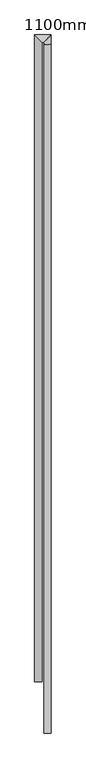
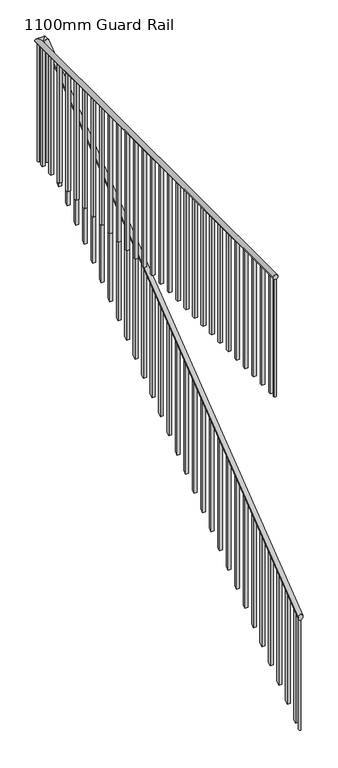
"""IFC4 building model written with IfcOpenShell, lengths in millimetres: railing geometry, 1100mm Guard Rail."""

from ifc_helpers import new_model, si_unit, point, frame, frame_2d, origin, place, context, project, spatial, polyline, circle_curve, ellipse_curve, trimmed, segment, composite_curve, outline, extrude, source, transform, mapped, element, save
from ifc_brep_helpers import plane_surface, cylinder_surface, advanced_brep


def railing_1100mm_guard_rail_51766e59(model_context):
    return source(origin(), model_context, "Body", "SolidModel", [
        advanced_brep(
        [(7413.6, -11825.0, 1268.4468381), (7373.6, -11825.0, 1268.4468381), (7413.6, -8068.1572105, 4180.0), (7373.6, -8068.1572105, 4180.0), (7373.6, -8060.0, 4180.0), (7413.6, -8020.0, 4180.0), (7323.6, -8020.0, 4180.0), (7363.6, -8060.0, 4180.0), (7323.6, -11545.0, 4180.0), (7363.6, -11545.0, 4180.0)],
        [
            (0, 1, ellipse_curve(frame((7393.6, -11825.0, 1268.4468381), z_axis=(0.0, -1.0, 0.0), x_axis=(0.0, 0.0, -1.0)), 25.3031619, 20.0)),
            (1, 0, ellipse_curve(frame((7393.6, -11825.0, 1268.4468381), z_axis=(0.0, -1.0, 0.0), x_axis=(0.0, 0.0, -1.0)), 25.3031619, 20.0)),
            (0, 2),
            (2, 3, ellipse_curve(frame((7393.6, -8068.1572105, 4180.0), z_axis=(0.0, -0.9461540710093745, -0.3237166568349356), x_axis=(0.0, 0.32371665683493556, -0.9461540710093745)), 21.1382064, 20.0)),
            (3, 1),
            (3, 2, ellipse_curve(frame((7393.6, -8068.1572105, 4180.0), z_axis=(0.0, -0.9461540710093745, -0.3237166568349356), x_axis=(0.0, 0.32371665683493556, -0.9461540710093745)), 21.1382064, 20.0)),
            (4, 5, ellipse_curve(frame((7393.6, -8040.0, 4180.0), z_axis=(-0.7071067811865475, 0.7071067811865475, 0.0), x_axis=(0.7071067811865476, 0.7071067811865474, 0.0)), 28.2842712, 20.0)),
            (5, 6),
            (6, 7, ellipse_curve(frame((7343.6, -8040.0, 4180.0), z_axis=(0.707106781186548, 0.7071067811865469, 0.0), x_axis=(0.7071067811865471, -0.7071067811865479, 0.0)), 28.2842712, 20.0)),
            (7, 4),
            (5, 4, ellipse_curve(frame((7393.6, -8040.0, 4180.0), z_axis=(-0.7071067811865475, 0.7071067811865475, 0.0), x_axis=(0.7071067811865476, 0.7071067811865474, 0.0)), 28.2842712, 20.0)),
            (7, 6, ellipse_curve(frame((7343.6, -8040.0, 4180.0), z_axis=(0.707106781186548, 0.7071067811865469, 0.0), x_axis=(0.7071067811865471, -0.7071067811865479, 0.0)), 28.2842712, 20.0)),
            (8, 9, circle_curve(frame((7343.6, -11545.0, 4180.0), z_axis=(0.0, -1.0, 0.0), x_axis=(1.0, 0.0, 0.0)), 20.0)),
            (9, 8, circle_curve(frame((7343.6, -11545.0, 4180.0), z_axis=(0.0, -1.0, 0.0), x_axis=(1.0, 0.0, 0.0)), 20.0)),
            (6, 8),
            (9, 7),
            (2, 5),
            (4, 3),
        ],
        [
            plane_surface(frame((7393.6, -11825.0, 1293.75), z_axis=(0.0, -1.0, 0.0), x_axis=(0.0, 0.0, 1.0))),
            cylinder_surface(frame((7393.6, -11812.7485667, 1277.941699), z_axis=(0.0, -0.7904150521752251, -0.612571665435838), x_axis=(-1.0, 0.0, 0.0)), 20.0),
            cylinder_surface(frame((7393.6, -8040.0, 4180.0), z_axis=(1.0, 0.0, 0.0), x_axis=(0.0, -1.0, 0.0)), 20.0),
            plane_surface(frame((7343.6, -11545.0, 4200.0), z_axis=(0.0, -1.0, 0.0), x_axis=(0.0, 0.0, -1.0))),
            cylinder_surface(frame((7343.6, -8040.0, 4180.0), z_axis=(0.0, 1.0, 0.0), x_axis=(1.0, 0.0, 0.0)), 20.0),
            cylinder_surface(frame((7393.6, -8075.0, 4180.0), z_axis=(0.0, -1.0, 0.0), x_axis=(-1.0, 0.0, 0.0)), 20.0),
        ],
        [
            (0, [[1, 2]]),
            (1, [[-1, 3, 4, 5]]),
            (1, [[-2, -5, 6, -3]]),
            (2, [[7, 8, 9, 10]]),
            (2, [[11, -10, 12, -8]]),
            (3, [[13, 14]]),
            (4, [[-9, 15, -14, 16]]),
            (4, [[-12, -16, -13, -15]]),
            (5, [[-4, 17, -7, 18]]),
            (5, [[-6, -18, -11, -17]]),
        ],
    ),
        extrude(outline(polyline([(7356.1, -11465.0), (7356.1, -11490.0), (7331.1, -11490.0), (7331.1, -11465.0), (7356.1, -11465.0)])), frame((0.0, 0.0, 3100.0), z_axis=(0.0, 0.0, 1.0), x_axis=(1.0, 0.0, 0.0)), (0.0, 0.0, 1.0), 1060.0),
        extrude(outline(polyline([(7356.1, -11340.0), (7356.1, -11365.0), (7331.1, -11365.0), (7331.1, -11340.0), (7356.1, -11340.0)])), frame((0.0, 0.0, 3100.0), z_axis=(0.0, 0.0, 1.0), x_axis=(1.0, 0.0, 0.0)), (0.0, 0.0, 1.0), 1060.0),
        extrude(outline(polyline([(7356.1, -11215.0), (7356.1, -11240.0), (7331.1, -11240.0), (7331.1, -11215.0), (7356.1, -11215.0)])), frame((0.0, 0.0, 3100.0), z_axis=(0.0, 0.0, 1.0), x_axis=(1.0, 0.0, 0.0)), (0.0, 0.0, 1.0), 1060.0),
        extrude(outline(polyline([(7356.1, -11090.0), (7356.1, -11115.0), (7331.1, -11115.0), (7331.1, -11090.0), (7356.1, -11090.0)])), frame((0.0, 0.0, 3100.0), z_axis=(0.0, 0.0, 1.0), x_axis=(1.0, 0.0, 0.0)), (0.0, 0.0, 1.0), 1060.0),
        extrude(outline(polyline([(7356.1, -10965.0), (7356.1, -10990.0), (7331.1, -10990.0), (7331.1, -10965.0), (7356.1, -10965.0)])), frame((0.0, 0.0, 3100.0), z_axis=(0.0, 0.0, 1.0), x_axis=(1.0, 0.0, 0.0)), (0.0, 0.0, 1.0), 1060.0),
        extrude(outline(polyline([(7356.1, -10840.0), (7356.1, -10865.0), (7331.1, -10865.0), (7331.1, -10840.0), (7356.1, -10840.0)])), frame((0.0, 0.0, 3100.0), z_axis=(0.0, 0.0, 1.0), x_axis=(1.0, 0.0, 0.0)), (0.0, 0.0, 1.0), 1060.0),
        extrude(outline(polyline([(7356.1, -10715.0), (7356.1, -10740.0), (7331.1, -10740.0), (7331.1, -10715.0), (7356.1, -10715.0)])), frame((0.0, 0.0, 3100.0), z_axis=(0.0, 0.0, 1.0), x_axis=(1.0, 0.0, 0.0)), (0.0, 0.0, 1.0), 1060.0),
        extrude(outline(polyline([(7356.1, -10590.0), (7356.1, -10615.0), (7331.1, -10615.0), (7331.1, -10590.0), (7356.1, -10590.0)])), frame((0.0, 0.0, 3100.0), z_axis=(0.0, 0.0, 1.0), x_axis=(1.0, 0.0, 0.0)), (0.0, 0.0, 1.0), 1060.0),
        extrude(outline(polyline([(7356.1, -10465.0), (7356.1, -10490.0), (7331.1, -10490.0), (7331.1, -10465.0), (7356.1, -10465.0)])), frame((0.0, 0.0, 3100.0), z_axis=(0.0, 0.0, 1.0), x_axis=(1.0, 0.0, 0.0)), (0.0, 0.0, 1.0), 1060.0),
        extrude(outline(polyline([(7356.1, -10340.0), (7356.1, -10365.0), (7331.1, -10365.0), (7331.1, -10340.0), (7356.1, -10340.0)])), frame((0.0, 0.0, 3100.0), z_axis=(0.0, 0.0, 1.0), x_axis=(1.0, 0.0, 0.0)), (0.0, 0.0, 1.0), 1060.0),
        extrude(outline(polyline([(7356.1, -10215.0), (7356.1, -10240.0), (7331.1, -10240.0), (7331.1, -10215.0), (7356.1, -10215.0)])), frame((0.0, 0.0, 3100.0), z_axis=(0.0, 0.0, 1.0), x_axis=(1.0, 0.0, 0.0)), (0.0, 0.0, 1.0), 1060.0),
        extrude(outline(polyline([(7356.1, -10090.0), (7356.1, -10115.0), (7331.1, -10115.0), (7331.1, -10090.0), (7356.1, -10090.0)])), frame((0.0, 0.0, 3100.0), z_axis=(0.0, 0.0, 1.0), x_axis=(1.0, 0.0, 0.0)), (0.0, 0.0, 1.0), 1060.0),
        extrude(outline(polyline([(7356.1, -9965.0), (7356.1, -9990.0), (7331.1, -9990.0), (7331.1, -9965.0), (7356.1, -9965.0)])), frame((0.0, 0.0, 3100.0), z_axis=(0.0, 0.0, 1.0), x_axis=(1.0, 0.0, 0.0)), (0.0, 0.0, 1.0), 1060.0),
        extrude(outline(polyline([(7356.1, -9840.0), (7356.1, -9865.0), (7331.1, -9865.0), (7331.1, -9840.0), (7356.1, -9840.0)])), frame((0.0, 0.0, 3100.0), z_axis=(0.0, 0.0, 1.0), x_axis=(1.0, 0.0, 0.0)), (0.0, 0.0, 1.0), 1060.0),
        extrude(outline(polyline([(7356.1, -9715.0), (7356.1, -9740.0), (7331.1, -9740.0), (7331.1, -9715.0), (7356.1, -9715.0)])), frame((0.0, 0.0, 3100.0), z_axis=(0.0, 0.0, 1.0), x_axis=(1.0, 0.0, 0.0)), (0.0, 0.0, 1.0), 1060.0),
        extrude(outline(polyline([(7356.1, -9590.0), (7356.1, -9615.0), (7331.1, -9615.0), (7331.1, -9590.0), (7356.1, -9590.0)])), frame((0.0, 0.0, 3100.0), z_axis=(0.0, 0.0, 1.0), x_axis=(1.0, 0.0, 0.0)), (0.0, 0.0, 1.0), 1060.0),
        extrude(outline(polyline([(7356.1, -9465.0), (7356.1, -9490.0), (7331.1, -9490.0), (7331.1, -9465.0), (7356.1, -9465.0)])), frame((0.0, 0.0, 3100.0), z_axis=(0.0, 0.0, 1.0), x_axis=(1.0, 0.0, 0.0)), (0.0, 0.0, 1.0), 1060.0),
        extrude(outline(polyline([(7356.1, -9340.0), (7356.1, -9365.0), (7331.1, -9365.0), (7331.1, -9340.0), (7356.1, -9340.0)])), frame((0.0, 0.0, 3100.0), z_axis=(0.0, 0.0, 1.0), x_axis=(1.0, 0.0, 0.0)), (0.0, 0.0, 1.0), 1060.0),
        extrude(outline(polyline([(7356.1, -9215.0), (7356.1, -9240.0), (7331.1, -9240.0), (7331.1, -9215.0), (7356.1, -9215.0)])), frame((0.0, 0.0, 3100.0), z_axis=(0.0, 0.0, 1.0), x_axis=(1.0, 0.0, 0.0)), (0.0, 0.0, 1.0), 1060.0),
        extrude(outline(polyline([(7356.1, -9090.0), (7356.1, -9115.0), (7331.1, -9115.0), (7331.1, -9090.0), (7356.1, -9090.0)])), frame((0.0, 0.0, 3100.0), z_axis=(0.0, 0.0, 1.0), x_axis=(1.0, 0.0, 0.0)), (0.0, 0.0, 1.0), 1060.0),
        extrude(outline(polyline([(7356.1, -8965.0), (7356.1, -8990.0), (7331.1, -8990.0), (7331.1, -8965.0), (7356.1, -8965.0)])), frame((0.0, 0.0, 3100.0), z_axis=(0.0, 0.0, 1.0), x_axis=(1.0, 0.0, 0.0)), (0.0, 0.0, 1.0), 1060.0),
        extrude(outline(polyline([(7356.1, -8840.0), (7356.1, -8865.0), (7331.1, -8865.0), (7331.1, -8840.0), (7356.1, -8840.0)])), frame((0.0, 0.0, 3100.0), z_axis=(0.0, 0.0, 1.0), x_axis=(1.0, 0.0, 0.0)), (0.0, 0.0, 1.0), 1060.0),
        extrude(outline(polyline([(7356.1, -8715.0), (7356.1, -8740.0), (7331.1, -8740.0), (7331.1, -8715.0), (7356.1, -8715.0)])), frame((0.0, 0.0, 3100.0), z_axis=(0.0, 0.0, 1.0), x_axis=(1.0, 0.0, 0.0)), (0.0, 0.0, 1.0), 1060.0),
        extrude(outline(polyline([(7356.1, -8590.0), (7356.1, -8615.0), (7331.1, -8615.0), (7331.1, -8590.0), (7356.1, -8590.0)])), frame((0.0, 0.0, 3100.0), z_axis=(0.0, 0.0, 1.0), x_axis=(1.0, 0.0, 0.0)), (0.0, 0.0, 1.0), 1060.0),
        extrude(outline(polyline([(7356.1, -8465.0), (7356.1, -8490.0), (7331.1, -8490.0), (7331.1, -8465.0), (7356.1, -8465.0)])), frame((0.0, 0.0, 3100.0), z_axis=(0.0, 0.0, 1.0), x_axis=(1.0, 0.0, 0.0)), (0.0, 0.0, 1.0), 1060.0),
        extrude(outline(polyline([(7356.1, -8340.0), (7356.1, -8365.0), (7331.1, -8365.0), (7331.1, -8340.0), (7356.1, -8340.0)])), frame((0.0, 0.0, 3100.0), z_axis=(0.0, 0.0, 1.0), x_axis=(1.0, 0.0, 0.0)), (0.0, 0.0, 1.0), 1060.0),
        extrude(outline(polyline([(7356.1, -8215.0), (7356.1, -8240.0), (7331.1, -8240.0), (7331.1, -8215.0), (7356.1, -8215.0)])), frame((0.0, 0.0, 3100.0), z_axis=(0.0, 0.0, 1.0), x_axis=(1.0, 0.0, 0.0)), (0.0, 0.0, 1.0), 1060.0),
        extrude(outline(polyline([(7356.1, -8090.0), (7356.1, -8115.0), (7331.1, -8115.0), (7331.1, -8090.0), (7356.1, -8090.0)])), frame((0.0, 0.0, 3100.0), z_axis=(0.0, 0.0, 1.0), x_axis=(1.0, 0.0, 0.0)), (0.0, 0.0, 1.0), 1060.0),
        extrude(outline(polyline([(-8150.0, 4091.2686763), (-8125.0, 4110.6436763), (-8125.0, 3100.0), (-8150.0, 3100.0), (-8150.0, 4091.2686763)])), frame((7381.1, 0.0, 0.0), z_axis=(1.0, 0.0, 0.0), x_axis=(0.0, 1.0, 0.0)), (0.0, 0.0, 1.0), 25.0),
        extrude(outline(polyline([(-8275.0, 3994.3936763), (-8250.0, 4013.7686763), (-8250.0, 3016.946707), (-8275.0, 2997.571707), (-8275.0, 3994.3936763)])), frame((7381.1, 0.0, 0.0), z_axis=(1.0, 0.0, 0.0), x_axis=(0.0, 1.0, 0.0)), (0.0, 0.0, 1.0), 25.0),
        extrude(outline(polyline([(-8400.0, 3897.5186763), (-8375.0, 3916.8936763), (-8375.0, 2920.071707), (-8400.0, 2900.696707), (-8400.0, 3897.5186763)])), frame((7381.1, 0.0, 0.0), z_axis=(1.0, 0.0, 0.0), x_axis=(0.0, 1.0, 0.0)), (0.0, 0.0, 1.0), 25.0),
        extrude(outline(polyline([(-8525.0, 3800.6436763), (-8500.0, 3820.0186763), (-8500.0, 2823.196707), (-8525.0, 2803.821707), (-8525.0, 3800.6436763)])), frame((7381.1, 0.0, 0.0), z_axis=(1.0, 0.0, 0.0), x_axis=(0.0, 1.0, 0.0)), (0.0, 0.0, 1.0), 25.0),
        extrude(outline(polyline([(-8650.0, 3703.7686763), (-8625.0, 3723.1436763), (-8625.0, 2726.321707), (-8650.0, 2706.946707), (-8650.0, 3703.7686763)])), frame((7381.1, 0.0, 0.0), z_axis=(1.0, 0.0, 0.0), x_axis=(0.0, 1.0, 0.0)), (0.0, 0.0, 1.0), 25.0),
        extrude(outline(polyline([(-8775.0, 3606.8936763), (-8750.0, 3626.2686763), (-8750.0, 2629.446707), (-8775.0, 2610.071707), (-8775.0, 3606.8936763)])), frame((7381.1, 0.0, 0.0), z_axis=(1.0, 0.0, 0.0), x_axis=(0.0, 1.0, 0.0)), (0.0, 0.0, 1.0), 25.0),
        extrude(outline(polyline([(-8900.0, 3510.0186763), (-8875.0, 3529.3936763), (-8875.0, 2532.571707), (-8900.0, 2513.196707), (-8900.0, 3510.0186763)])), frame((7381.1, 0.0, 0.0), z_axis=(1.0, 0.0, 0.0), x_axis=(0.0, 1.0, 0.0)), (0.0, 0.0, 1.0), 25.0),
        extrude(outline(polyline([(-9025.0, 3413.1436763), (-9000.0, 3432.5186763), (-9000.0, 2435.696707), (-9025.0, 2416.321707), (-9025.0, 3413.1436763)])), frame((7381.1, 0.0, 0.0), z_axis=(1.0, 0.0, 0.0), x_axis=(0.0, 1.0, 0.0)), (0.0, 0.0, 1.0), 25.0),
        extrude(outline(polyline([(-9150.0, 3316.2686763), (-9125.0, 3335.6436763), (-9125.0, 2338.821707), (-9150.0, 2319.446707), (-9150.0, 3316.2686763)])), frame((7381.1, 0.0, 0.0), z_axis=(1.0, 0.0, 0.0), x_axis=(0.0, 1.0, 0.0)), (0.0, 0.0, 1.0), 25.0),
        extrude(outline(polyline([(-9275.0, 3219.3936763), (-9250.0, 3238.7686763), (-9250.0, 2241.946707), (-9275.0, 2222.571707), (-9275.0, 3219.3936763)])), frame((7381.1, 0.0, 0.0), z_axis=(1.0, 0.0, 0.0), x_axis=(0.0, 1.0, 0.0)), (0.0, 0.0, 1.0), 25.0),
        extrude(outline(polyline([(-9400.0, 3122.5186763), (-9375.0, 3141.8936763), (-9375.0, 2145.071707), (-9400.0, 2125.696707), (-9400.0, 3122.5186763)])), frame((7381.1, 0.0, 0.0), z_axis=(1.0, 0.0, 0.0), x_axis=(0.0, 1.0, 0.0)), (0.0, 0.0, 1.0), 25.0),
        extrude(outline(polyline([(-9525.0, 3025.6436763), (-9500.0, 3045.0186763), (-9500.0, 2048.196707), (-9525.0, 2028.821707), (-9525.0, 3025.6436763)])), frame((7381.1, 0.0, 0.0), z_axis=(1.0, 0.0, 0.0), x_axis=(0.0, 1.0, 0.0)), (0.0, 0.0, 1.0), 25.0),
        extrude(outline(polyline([(-9650.0, 2928.7686763), (-9625.0, 2948.1436763), (-9625.0, 1951.321707), (-9650.0, 1931.946707), (-9650.0, 2928.7686763)])), frame((7381.1, 0.0, 0.0), z_axis=(1.0, 0.0, 0.0), x_axis=(0.0, 1.0, 0.0)), (0.0, 0.0, 1.0), 25.0),
        extrude(outline(polyline([(-9775.0, 2831.8936763), (-9750.0, 2851.2686763), (-9750.0, 1854.446707), (-9775.0, 1835.071707), (-9775.0, 2831.8936763)])), frame((7381.1, 0.0, 0.0), z_axis=(1.0, 0.0, 0.0), x_axis=(0.0, 1.0, 0.0)), (0.0, 0.0, 1.0), 25.0),
        extrude(outline(polyline([(-9900.0, 2735.0186763), (-9875.0, 2754.3936763), (-9875.0, 1757.571707), (-9900.0, 1738.196707), (-9900.0, 2735.0186763)])), frame((7381.1, 0.0, 0.0), z_axis=(1.0, 0.0, 0.0), x_axis=(0.0, 1.0, 0.0)), (0.0, 0.0, 1.0), 25.0),
        extrude(outline(polyline([(-10025.0, 2638.1436763), (-10000.0, 2657.5186763), (-10000.0, 1660.696707), (-10025.0, 1641.321707), (-10025.0, 2638.1436763)])), frame((7381.1, 0.0, 0.0), z_axis=(1.0, 0.0, 0.0), x_axis=(0.0, 1.0, 0.0)), (0.0, 0.0, 1.0), 25.0),
        extrude(outline(polyline([(-10150.0, 2541.2686763), (-10125.0, 2560.6436763), (-10125.0, 1563.821707), (-10150.0, 1544.446707), (-10150.0, 2541.2686763)])), frame((7381.1, 0.0, 0.0), z_axis=(1.0, 0.0, 0.0), x_axis=(0.0, 1.0, 0.0)), (0.0, 0.0, 1.0), 25.0),
        extrude(outline(polyline([(-10275.0, 2444.3936763), (-10250.0, 2463.7686763), (-10250.0, 1466.946707), (-10275.0, 1447.571707), (-10275.0, 2444.3936763)])), frame((7381.1, 0.0, 0.0), z_axis=(1.0, 0.0, 0.0), x_axis=(0.0, 1.0, 0.0)), (0.0, 0.0, 1.0), 25.0),
        extrude(outline(polyline([(-10400.0, 2347.5186763), (-10375.0, 2366.8936763), (-10375.0, 1370.071707), (-10400.0, 1350.696707), (-10400.0, 2347.5186763)])), frame((7381.1, 0.0, 0.0), z_axis=(1.0, 0.0, 0.0), x_axis=(0.0, 1.0, 0.0)), (0.0, 0.0, 1.0), 25.0),
        extrude(outline(polyline([(-10525.0, 2250.6436763), (-10500.0, 2270.0186763), (-10500.0, 1273.196707), (-10525.0, 1253.821707), (-10525.0, 2250.6436763)])), frame((7381.1, 0.0, 0.0), z_axis=(1.0, 0.0, 0.0), x_axis=(0.0, 1.0, 0.0)), (0.0, 0.0, 1.0), 25.0),
        extrude(outline(polyline([(-10650.0, 2153.7686763), (-10625.0, 2173.1436763), (-10625.0, 1176.321707), (-10650.0, 1156.946707), (-10650.0, 2153.7686763)])), frame((7381.1, 0.0, 0.0), z_axis=(1.0, 0.0, 0.0), x_axis=(0.0, 1.0, 0.0)), (0.0, 0.0, 1.0), 25.0),
        extrude(outline(polyline([(-10775.0, 2056.8936763), (-10750.0, 2076.2686763), (-10750.0, 1079.446707), (-10775.0, 1060.071707), (-10775.0, 2056.8936763)])), frame((7381.1, 0.0, 0.0), z_axis=(1.0, 0.0, 0.0), x_axis=(0.0, 1.0, 0.0)), (0.0, 0.0, 1.0), 25.0),
        extrude(outline(polyline([(-10900.0, 1960.0186763), (-10875.0, 1979.3936763), (-10875.0, 982.571707), (-10900.0, 963.196707), (-10900.0, 1960.0186763)])), frame((7381.1, 0.0, 0.0), z_axis=(1.0, 0.0, 0.0), x_axis=(0.0, 1.0, 0.0)), (0.0, 0.0, 1.0), 25.0),
        extrude(outline(polyline([(-11025.0, 1863.1436763), (-11000.0, 1882.5186763), (-11000.0, 885.696707), (-11025.0, 866.321707), (-11025.0, 1863.1436763)])), frame((7381.1, 0.0, 0.0), z_axis=(1.0, 0.0, 0.0), x_axis=(0.0, 1.0, 0.0)), (0.0, 0.0, 1.0), 25.0),
        extrude(outline(polyline([(-11150.0, 1766.2686763), (-11125.0, 1785.6436763), (-11125.0, 788.821707), (-11150.0, 769.446707), (-11150.0, 1766.2686763)])), frame((7381.1, 0.0, 0.0), z_axis=(1.0, 0.0, 0.0), x_axis=(0.0, 1.0, 0.0)), (0.0, 0.0, 1.0), 25.0),
        extrude(outline(polyline([(-11275.0, 1669.3936763), (-11250.0, 1688.7686763), (-11250.0, 691.946707), (-11275.0, 672.571707), (-11275.0, 1669.3936763)])), frame((7381.1, 0.0, 0.0), z_axis=(1.0, 0.0, 0.0), x_axis=(0.0, 1.0, 0.0)), (0.0, 0.0, 1.0), 25.0),
        extrude(outline(polyline([(-11400.0, 1572.5186763), (-11375.0, 1591.8936763), (-11375.0, 595.071707), (-11400.0, 575.696707), (-11400.0, 1572.5186763)])), frame((7381.1, 0.0, 0.0), z_axis=(1.0, 0.0, 0.0), x_axis=(0.0, 1.0, 0.0)), (0.0, 0.0, 1.0), 25.0),
        extrude(outline(polyline([(-11525.0, 1475.6436763), (-11500.0, 1495.0186763), (-11500.0, 498.196707), (-11525.0, 478.821707), (-11525.0, 1475.6436763)])), frame((7381.1, 0.0, 0.0), z_axis=(1.0, 0.0, 0.0), x_axis=(0.0, 1.0, 0.0)), (0.0, 0.0, 1.0), 25.0),
        extrude(outline(polyline([(-11650.0, 1378.7686763), (-11625.0, 1398.1436763), (-11625.0, 401.321707), (-11650.0, 381.946707), (-11650.0, 1378.7686763)])), frame((7381.1, 0.0, 0.0), z_axis=(1.0, 0.0, 0.0), x_axis=(0.0, 1.0, 0.0)), (0.0, 0.0, 1.0), 25.0),
        extrude(outline(polyline([(-11775.0, 1281.8936763), (-11750.0, 1301.2686763), (-11750.0, 304.446707), (-11775.0, 285.071707), (-11775.0, 1281.8936763)])), frame((7381.1, 0.0, 0.0), z_axis=(1.0, 0.0, 0.0), x_axis=(0.0, 1.0, 0.0)), (0.0, 0.0, 1.0), 25.0),
        extrude(outline(composite_curve([segment(trimmed(circle_curve(frame_2d((7343.6, -8040.0)), 10.0), [point((7343.6, -8030.0))], [point((7343.6, -8050.0))], False, "CARTESIAN"), True, "CONTINUOUS"), segment(trimmed(circle_curve(frame_2d((7343.6, -8040.0)), 10.0), [point((7343.6, -8050.0))], [point((7343.6, -8030.0))], False, "CARTESIAN"), True, "CONTINUOUS")], self_intersect=False)), frame((0.0, 0.0, 3100.0), z_axis=(0.0, 0.0, 1.0), x_axis=(1.0, 0.0, 0.0)), (0.0, 0.0, 1.0), 1060.0),
        extrude(outline(composite_curve([segment(trimmed(circle_curve(frame_2d((7393.6, -8040.0)), 10.0), [point((7403.6, -8040.0))], [point((7383.6, -8040.0))], False, "CARTESIAN"), True, "CONTINUOUS"), segment(trimmed(circle_curve(frame_2d((7393.6, -8040.0)), 10.0), [point((7383.6, -8040.0))], [point((7403.6, -8040.0))], False, "CARTESIAN"), True, "CONTINUOUS")], self_intersect=False)), frame((0.0, 0.0, 3100.0), z_axis=(0.0, 0.0, 1.0), x_axis=(1.0, 0.0, 0.0)), (0.0, 0.0, 1.0), 1060.0),
        extrude(outline(composite_curve([segment(trimmed(circle_curve(frame_2d((7393.6, -8075.0)), 10.0), [point((7403.6, -8075.0))], [point((7383.6, -8075.0))], False, "CARTESIAN"), True, "CONTINUOUS"), segment(trimmed(circle_curve(frame_2d((7393.6, -8075.0)), 10.0), [point((7383.6, -8075.0))], [point((7403.6, -8075.0))], False, "CARTESIAN"), True, "CONTINUOUS")], self_intersect=False)), frame((0.0, 0.0, 3100.0), z_axis=(0.0, 0.0, 1.0), x_axis=(1.0, 0.0, 0.0)), (0.0, 0.0, 1.0), 1060.0),
        extrude(outline(composite_curve([segment(trimmed(circle_curve(frame_2d((7343.6, -11532.5)), 10.0), [point((7333.6, -11532.5))], [point((7353.6, -11532.5))], False, "CARTESIAN"), True, "CONTINUOUS"), segment(trimmed(circle_curve(frame_2d((7343.6, -11532.5)), 10.0), [point((7353.6, -11532.5))], [point((7333.6, -11532.5))], False, "CARTESIAN"), True, "CONTINUOUS")], self_intersect=False)), frame((0.0, 0.0, 3100.0), z_axis=(0.0, 0.0, 1.0), x_axis=(1.0, 0.0, 0.0)), (0.0, 0.0, 1.0), 1060.0),
        advanced_brep(
        [(7383.6, -11812.5, 1252.8311763), (7403.6, -11812.5, 1252.8311763), (7403.6, -11812.5, 256.009207), (7383.6, -11812.5, 256.009207)],
        [
            (0, 1, ellipse_curve(frame((7393.6, -11812.5, 1252.8311763), z_axis=(0.0, 0.6125716654358373, -0.7904150521752257), x_axis=(0.0, 0.7904150521752258, 0.6125716654358372)), 12.6515809, 10.0)),
            (1, 2),
            (2, 3, ellipse_curve(frame((7393.6, -11812.5, 256.009207), z_axis=(0.0, -0.6125716654358382, 0.790415052175225), x_axis=(0.0, 0.790415052175225, 0.612571665435838)), 12.6515809, 10.0)),
            (3, 0),
            (3, 2, ellipse_curve(frame((7393.6, -11812.5, 256.009207), z_axis=(0.0, -0.6125716654358382, 0.790415052175225), x_axis=(0.0, 0.790415052175225, 0.612571665435838)), 12.6515809, 10.0)),
            (1, 0, ellipse_curve(frame((7393.6, -11812.5, 1252.8311763), z_axis=(0.0, 0.6125716654358373, -0.7904150521752257), x_axis=(0.0, 0.7904150521752258, 0.6125716654358372)), 12.6515809, 10.0)),
        ],
        [
            cylinder_surface(frame((7393.6, -11812.5, 156.009207), z_axis=(0.0, 0.0, 1.0), x_axis=(1.0, 0.0, 0.0)), 10.0),
            plane_surface(frame((7413.6, -11792.5, 1268.3311763), z_axis=(0.0, -0.6125716654358373, 0.7904150521752257), x_axis=(-1.0, 0.0, 0.0))),
            plane_surface(frame((7413.6, -11832.5, 240.509207), z_axis=(0.0, 0.6125716654358382, -0.790415052175225), x_axis=(-1.0, 0.0, 0.0))),
        ],
        [
            (0, [[1, 2, 3, 4]]),
            (0, [[5, -2, 6, -4]]),
            (1, [[-6, -1]]),
            (2, [[-5, -3]]),
        ],
    ),
    ])


if __name__ == "__main__":
    model = new_model("IFC4")
    model_context = context("Model", 3, world=origin())
    ifc_project = project(units=[si_unit("LENGTHUNIT", "METRE", prefix="MILLI")], contexts=[model_context])
    site = spatial("IfcSite", under=ifc_project)
    building = spatial("IfcBuilding", under=site)
    placement = place(None, origin())
    railing_1100mm_guard_rail_shape = railing_1100mm_guard_rail_51766e59(model_context)
    element("IfcRailing", 1, ObjectType="1100mm Guard Rail", at=placement, inside=building, context=model_context, shape_type="MappedRepresentation", body=[
        mapped(railing_1100mm_guard_rail_shape, transform((0.0, 0.0, 0.0), x_axis=(1.0, 0.0, 0.0), y_axis=(0.0, 1.0, 0.0), z_axis=(0.0, 0.0, 1.0))),
    ])
    save(model, "model.ifc")
